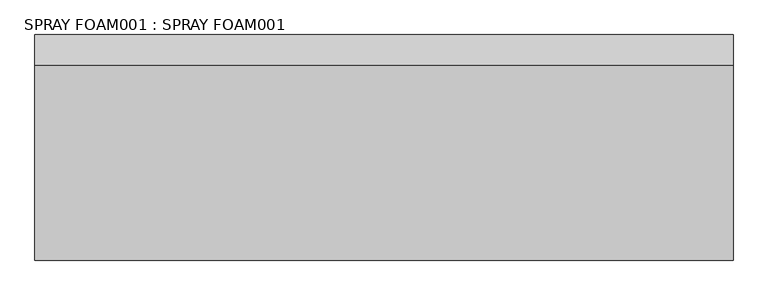
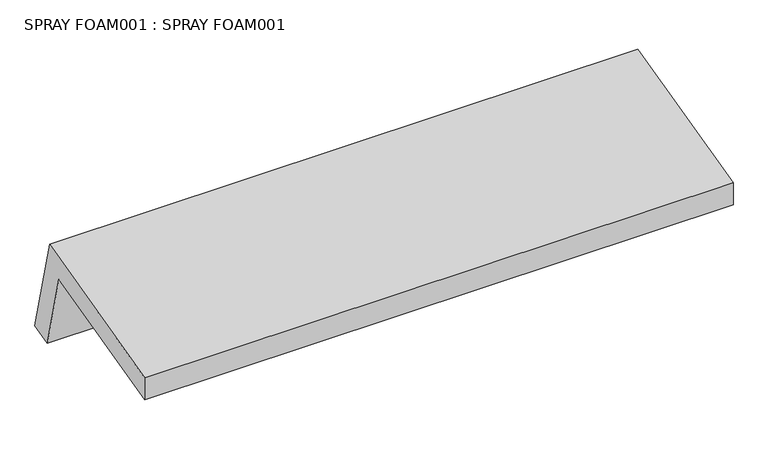
"""IFC4 building model written with IfcOpenShell, lengths in millimetres: proxy geometry, SPRAY FOAM001 : SPRAY FOAM001."""

from ifc_helpers import new_model, si_unit, frame, origin, place, context, project, spatial, polyline, outline, extrude, source, transform, mapped, element, save


def spray_foam001_spray_foam001_9babf991(model_context):
    return source(origin(), model_context, "Body", "SweptSolid", [
        extrude(outline(polyline([(8857.5938813, 43384.4932401), (9417.6229917, 43524.5643553), (9503.8912781, 43179.5873376), (9429.9539501, 43161.1560729), (9362.1861979, 43432.1515684), (8857.5938813, 43305.9459708), (8857.5938813, 43384.4932401)])), frame((3700.3883192, 0.0, 0.0), z_axis=(1.0, 0.0, 0.0), x_axis=(0.0, 1.0, 0.0)), (0.0, 0.0, 1.0), 2000.25),
    ])


if __name__ == "__main__":
    model = new_model("IFC4")
    model_context = context("Model", 3, world=origin())
    ifc_project = project(units=[si_unit("LENGTHUNIT", "METRE", prefix="MILLI")], contexts=[model_context])
    site = spatial("IfcSite", under=ifc_project)
    building = spatial("IfcBuilding", under=site)
    placement = place(None, origin())
    spray_foam001_spray_foam001_shape = spray_foam001_spray_foam001_9babf991(model_context)
    element("IfcBuildingElementProxy", 1, Name="SPRAY FOAM001 : SPRAY FOAM001", ObjectType="SPRAY FOAM001 : SPRAY FOAM001", at=placement, inside=building, context=model_context, shape_type="MappedRepresentation", body=[
        mapped(spray_foam001_spray_foam001_shape, transform((0.0, 0.0, 0.0), x_axis=(1.0, 0.0, 0.0), y_axis=(0.0, 1.0, 0.0), z_axis=(0.0, 0.0, 1.0))),
    ])
    save(model, "model.ifc")

# Revit data of these elements
# Type "SPRAY FOAM001 : SPRAY FOAM001"
#   NameOverride = "SPRAY FOAM001"
# Element 1 (IfcBuildingElementProxy, "SPRAY FOAM001 : SPRAY FOAM001")
#   Materials on its faces: "3\" POLYURETHANE SPRAY FOAM UNDER ROOF SUBSTRATE 3137"
# Materials
#   "3\" POLYURETHANE SPRAY FOAM UNDER ROOF SUBSTRATE 3137": class "Unassigned", colour RGB 193 227 245, transparency 0
